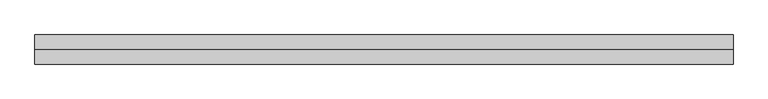
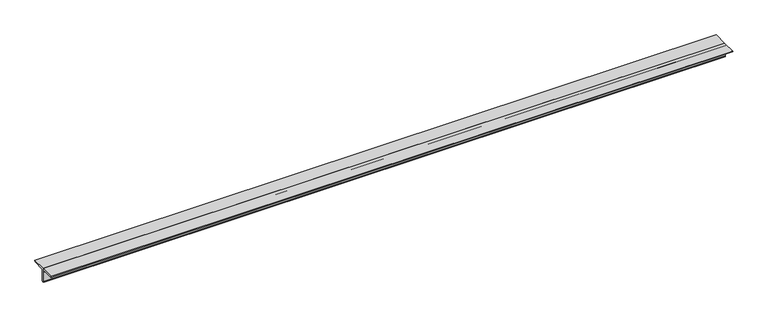
"""IFC4 building model written with IfcOpenShell, lengths in millimetres: member geometry, Steel Framing_2Ls_KS : H_SB_AR_S02_2Ls-100x100x10_VBR1."""

import ifcopenshell
import ifcopenshell.guid

model = None  # the IFC model being written
_history = None  # IfcOwnerHistory: only IFC2X3 demands one
_inside = {}  # id of a spatial element -> (the spatial element, [elements in it])
_under = {}  # id of a project, library or spatial element -> (it, [spatial elements below it])
_declared = {}  # id of a project -> (the project, [libraries it declares])
_typed = {}  # id of a type object -> (the type object, [elements of that type])
_made_of = {}  # id of a material, layer set ... -> (it, [elements and type objects made of it])


def new_model(schema):
    """Start an empty IFC model of exactly this schema.

    Asked for "IFC4X3", IfcOpenShell would pick the latest addendum, in which some entities
    have other attributes; the version numbers below select the first issue.
    IFC2X3 requires an IfcOwnerHistory on every rooted entity: one is made here for all.
    """
    global model, _history
    if schema == "IFC4X3":
        model = ifcopenshell.file(schema_version=(4, 3, 0, 0))
    else:
        model = ifcopenshell.file(schema=schema)
    _inside.clear()
    _under.clear()
    _declared.clear()
    _typed.clear()
    _made_of.clear()
    _history = None
    if model.schema == "IFC2X3":
        org = make("IfcOrganization", Name="unknown")
        user = make(
            "IfcPersonAndOrganization",
            ThePerson=make("IfcPerson", FamilyName="unknown"),
            TheOrganization=org,
        )
        app = make(
            "IfcApplication",
            ApplicationDeveloper=org,
            Version="unknown",
            ApplicationFullName="unknown",
            ApplicationIdentifier="unknown",
        )
        _history = make(
            "IfcOwnerHistory",
            OwningUser=user,
            OwningApplication=app,
            ChangeAction="ADDED",
            CreationDate=0,
        )
    return model


def make(cls, **values):
    """One entity of the class cls with the attributes given. An attribute that is None is left unset."""
    return model.create_entity(
        cls, **{name: value for name, value in values.items() if value is not None}
    )


def rooted(cls, **values):
    """An entity with a GlobalId (a new one), such as an element, a storey or a relation."""
    return make(cls, GlobalId=ifcopenshell.guid.new(), OwnerHistory=_history, **values)


def si_unit(unit_type, name, prefix=None):
    """IfcSIUnit, for example si_unit("LENGTHUNIT", "METRE", prefix="MILLI")."""
    return make("IfcSIUnit", UnitType=unit_type, Prefix=prefix, Name=name)


def assignment(units):
    """IfcUnitAssignment: the units of a project."""
    return None if units is None else make("IfcUnitAssignment", Units=units)


def point(xyz):
    """IfcCartesianPoint."""
    return None if xyz is None else make("IfcCartesianPoint", Coordinates=xyz)


def direction(xyz):
    """IfcDirection."""
    return None if xyz is None else make("IfcDirection", DirectionRatios=xyz)


def frame(location, z_axis=None, x_axis=None):
    """IfcAxis2Placement3D, a coordinate frame: its origin and axes. An axis left out is left unset."""
    return make(
        "IfcAxis2Placement3D",
        Location=point(location),
        Axis=direction(z_axis),
        RefDirection=direction(x_axis),
    )


def frame_2d(location, x_axis=None):
    """IfcAxis2Placement2D, a coordinate frame in the plane: its origin and x axis."""
    return make(
        "IfcAxis2Placement2D", Location=point(location), RefDirection=direction(x_axis)
    )


def origin():
    """The frame at (0, 0, 0) with its axes left unset."""
    return frame((0.0, 0.0, 0.0))


def place(relative_to, where):
    """IfcLocalPlacement: puts the frame where relative to a parent placement (None: the world)."""
    return make(
        "IfcLocalPlacement", PlacementRelTo=relative_to, RelativePlacement=where
    )


def context(
    kind, dimensions, precision=None, world=None, true_north=None, identifier=None
):
    """IfcGeometricRepresentationContext, for example the 3D "Model" context."""
    return make(
        "IfcGeometricRepresentationContext",
        ContextIdentifier=identifier,
        ContextType=kind,
        CoordinateSpaceDimension=dimensions,
        Precision=precision,
        WorldCoordinateSystem=world,
        TrueNorth=true_north,
    )


def project(units=None, contexts=None):
    """IfcProject with its units and contexts."""
    return rooted(
        "IfcProject",
        Name="project",
        RepresentationContexts=contexts,
        UnitsInContext=assignment(units),
    )


def spatial(cls, under=None, at=None, **own):
    """A site, building, storey or space (cls), placed at a placement, below another one or the project."""
    s = rooted(cls, ObjectPlacement=at, **own)
    if under is not None:
        _under.setdefault(under.id(), (under, []))[1].append(s)
    return s


def polyline(points):
    """IfcPolyline through the points."""
    return make("IfcPolyline", Points=[point(p) for p in points])


def circle_curve(where, radius):
    """IfcCircle in the frame where."""
    return make("IfcCircle", Position=where, Radius=radius)


def trimmed(basis, trim1, trim2, sense, master):
    """IfcTrimmedCurve: the piece of a basis curve between two trims."""
    return make(
        "IfcTrimmedCurve",
        BasisCurve=basis,
        Trim1=trim1,
        Trim2=trim2,
        SenseAgreement=sense,
        MasterRepresentation=master,
    )


def segment(curve, same_sense, transition):
    """IfcCompositeCurveSegment."""
    return make(
        "IfcCompositeCurveSegment",
        Transition=transition,
        SameSense=same_sense,
        ParentCurve=curve,
    )


def composite_curve(segments, self_intersect=None):
    """IfcCompositeCurve: segments joined end to end."""
    return make("IfcCompositeCurve", Segments=segments, SelfIntersect=self_intersect)


def outline(outer, holes=None, kind="AREA"):
    """IfcArbitraryClosedProfileDef: a profile drawn as a closed curve; with holes, ...WithVoids."""
    if holes is None:
        return make("IfcArbitraryClosedProfileDef", ProfileType=kind, OuterCurve=outer)
    return make(
        "IfcArbitraryProfileDefWithVoids",
        ProfileType=kind,
        OuterCurve=outer,
        InnerCurves=holes,
    )


def extrude(swept, where, along, depth):
    """IfcExtrudedAreaSolid: the profile swept, set in the frame where, extruded along a direction by depth."""
    return make(
        "IfcExtrudedAreaSolid",
        SweptArea=swept,
        Position=where,
        ExtrudedDirection=direction(along),
        Depth=depth,
    )


def shape(context_of_items, identifier, shape_type, items):
    """IfcShapeRepresentation: the items that make up one representation, for example the "Body"."""
    return make(
        "IfcShapeRepresentation",
        ContextOfItems=context_of_items,
        RepresentationIdentifier=identifier,
        RepresentationType=shape_type,
        Items=items,
    )


def source(mapping_origin, context_of_items, identifier, shape_type, items):
    """IfcRepresentationMap: a shape defined once, which mapped items show again and again."""
    return make(
        "IfcRepresentationMap",
        MappingOrigin=mapping_origin,
        MappedRepresentation=shape(context_of_items, identifier, shape_type, items),
    )


def transform(
    local_origin,
    x_axis=None,
    y_axis=None,
    z_axis=None,
    scale=None,
    scale2=None,
    scale3=None,
    uniform=True,
):
    """IfcCartesianTransformationOperator3D, or its non-uniform kind. x_axis, y_axis, z_axis: its Axis1, 2, 3."""
    if uniform:
        return make(
            "IfcCartesianTransformationOperator3D",
            Axis1=direction(x_axis),
            Axis2=direction(y_axis),
            LocalOrigin=point(local_origin),
            Scale=scale,
            Axis3=direction(z_axis),
        )
    return make(
        "IfcCartesianTransformationOperator3DnonUniform",
        Axis1=direction(x_axis),
        Axis2=direction(y_axis),
        LocalOrigin=point(local_origin),
        Scale=scale,
        Axis3=direction(z_axis),
        Scale2=scale2,
        Scale3=scale3,
    )


def mapped(mapping_source, mapping_target):
    """IfcMappedItem: shows the shape of a source again, moved by a transform."""
    return make(
        "IfcMappedItem", MappingSource=mapping_source, MappingTarget=mapping_target
    )


def made_of(thing, what):
    """Note that an element or type object is made of a material, layer set ...; save() writes the relation."""
    if what is not None:
        _made_of.setdefault(what.id(), (what, []))[1].append(thing)
    return thing


def element(
    cls,
    number,
    at=None,
    inside=None,
    cuts=None,
    type_object=None,
    material=None,
    context=None,
    identifier="Body",
    shape_type=None,
    held_by="IfcProductDefinitionShape",
    body=None,
    shapes=None,
    **own,
):
    """One element of the class cls, such as IfcWall. Its Tag is "e" and its number.

    at: its placement. inside: the storey or other place that contains it. cuts: it is an
    opening in that element (IfcRelVoidsElement). A single representation is given by context,
    identifier, shape_type and body (its items); several are given by shapes. held_by: the class
    of the entity that holds the representations. save() writes the other relations.
    """
    e = rooted(cls, Tag="e%d" % number, ObjectPlacement=at, **own)
    if body is not None:
        shapes = [shape(context, identifier, shape_type, body)]
    if shapes is not None:
        e.Representation = make(held_by, Representations=shapes)
    if inside is not None:
        _inside.setdefault(inside.id(), (inside, []))[1].append(e)
    if cuts is not None:
        rooted(
            "IfcRelVoidsElement", RelatingBuildingElement=cuts, RelatedOpeningElement=e
        )
    if type_object is not None:
        _typed.setdefault(type_object.id(), (type_object, []))[1].append(e)
    return made_of(e, material)


def aggregate(whole, parts):
    """IfcRelAggregates: a whole, such as a stair, and the parts it consists of."""
    return rooted("IfcRelAggregates", RelatingObject=whole, RelatedObjects=parts)


def save(model, path):
    """Write the relations noted so far, then the file.

    IfcRelAggregates (storeys below a building ...), IfcRelContainedInSpatialStructure (elements
    in a storey), IfcRelDefinesByType, IfcRelAssociatesMaterial and IfcRelDeclares: one each for
    every whole, place, type object, material and project.
    """
    for whole, parts in _under.values():
        aggregate(whole, parts)
    for where, things in _inside.values():
        rooted(
            "IfcRelContainedInSpatialStructure",
            RelatedElements=things,
            RelatingStructure=where,
        )
    for kind, things in _typed.values():
        rooted("IfcRelDefinesByType", RelatedObjects=things, RelatingType=kind)
    for what, things in _made_of.values():
        rooted("IfcRelAssociatesMaterial", RelatedObjects=things, RelatingMaterial=what)
    for by, libraries in _declared.values():
        rooted("IfcRelDeclares", RelatingContext=by, RelatedDefinitions=libraries)
    model.write(path)


def member_7977efe3(model_context):
    return source(origin(), model_context, "Body", "SweptSolid", [
        extrude(outline(composite_curve([segment(polyline([(0.0, 28.2), (100.0, 28.2)]), True, "CONTINUOUS"), segment(trimmed(circle_curve(frame_2d((90.0, 28.2)), 10.0), [point((100.0, 28.2))], [point((90.0, 18.2))], False, "CARTESIAN"), True, "CONTINUOUS"), segment(polyline([(90.0, 18.2), (20.0, 18.2)]), True, "CONTINUOUS"), segment(trimmed(circle_curve(frame_2d((20.0, 8.2)), 10.0), [point((20.0, 18.2))], [point((10.0, 8.2))], True, "CARTESIAN"), True, "CONTINUOUS"), segment(polyline([(10.0, 8.2), (10.0, -61.8)]), True, "CONTINUOUS"), segment(trimmed(circle_curve(frame_2d((0.0, -61.8)), 10.0), [point((10.0, -61.8))], [point((0.0, -71.8))], False, "CARTESIAN"), True, "CONTINUOUS"), segment(polyline([(0.0, -71.8), (0.0, 28.2)]), True, "CONTINUOUS")], self_intersect=False)), frame((-2442.577408, 0.0, 0.0), z_axis=(1.0, 0.0, 0.0), x_axis=(0.0, 1.0, 0.0)), (0.0, 0.0, 1.0), 4793.1814616),
        extrude(outline(composite_curve([segment(polyline([(0.0, 28.2), (0.0, -71.8)]), True, "CONTINUOUS"), segment(trimmed(circle_curve(frame_2d((0.0, -61.8)), 10.0), [point((0.0, -71.8))], [point((-10.0, -61.8))], False, "CARTESIAN"), True, "CONTINUOUS"), segment(polyline([(-10.0, -61.8), (-10.0, 8.2)]), True, "CONTINUOUS"), segment(trimmed(circle_curve(frame_2d((-20.0, 8.2)), 10.0), [point((-10.0, 8.2))], [point((-20.0, 18.2))], True, "CARTESIAN"), True, "CONTINUOUS"), segment(polyline([(-20.0, 18.2), (-90.0, 18.2)]), True, "CONTINUOUS"), segment(trimmed(circle_curve(frame_2d((-90.0, 28.2)), 10.0), [point((-90.0, 18.2))], [point((-100.0, 28.2))], False, "CARTESIAN"), True, "CONTINUOUS"), segment(polyline([(-100.0, 28.2), (0.0, 28.2)]), True, "CONTINUOUS")], self_intersect=False)), frame((-2442.577408, 0.0, 0.0), z_axis=(1.0, 0.0, 0.0), x_axis=(0.0, 1.0, 0.0)), (0.0, 0.0, 1.0), 4793.1814616),
    ])


if __name__ == "__main__":
    model = new_model("IFC4")
    model_context = context("Model", 3, world=origin())
    ifc_project = project(units=[si_unit("LENGTHUNIT", "METRE", prefix="MILLI")], contexts=[model_context])
    site = spatial("IfcSite", under=ifc_project)
    building = spatial("IfcBuilding", under=site)
    placement = place(None, origin())
    member_shape = member_7977efe3(model_context)
    element("IfcMember", 1, ObjectType="Steel Framing_2Ls_KS : H_SB_AR_S02_2Ls-100x100x10_VBR1", at=placement, inside=building, context=model_context, shape_type="MappedRepresentation", body=[
        mapped(member_shape, transform((0.0, 0.0, 0.0), x_axis=(1.0, 0.0, 0.0), y_axis=(0.0, 1.0, 0.0), z_axis=(0.0, 0.0, 1.0))),
    ])
    save(model, "model.ifc")

# Revit data of these elements
# Type "Steel Framing_2Ls_KS : H_SB_AR_S02_2Ls-100x100x10_VBR1"
#   Type Comments = "MAIN"
#   Type Mark = "VBR1"
#   H_SectionID = "2Ls-100x100x10"
#   Assembly Code = "B10"
#   Legs = "LLBB"
#   H_Ratio for Additional Steel Plate = 0.2
#   W = 0
#   Perimeter = 0.80 m²/m
#   Nominal Weight = 29.80 kgf/m
#   Length [instance default] = 1524 mm
#   Space = 0 mm
#   b = 100 mm
#   d = 100 mm
#   t = 10 mm
#   y = 28.2 mm
#   A = 0.0038 m²
#   Structural Material [instance default] = Steel, 45-345
# Element 1 (IfcMember, "Steel Framing_2Ls_KS : H_SB_AR_S02_2Ls-100x100x10_VBR1")
#   Materials on its faces: "Steel, 45-345"
# Materials
#   "Steel, 45-345": class "Metal", colour RGB 189 187 185, transparency 0, Description = "Steel 345 MPa", Cost = 0
